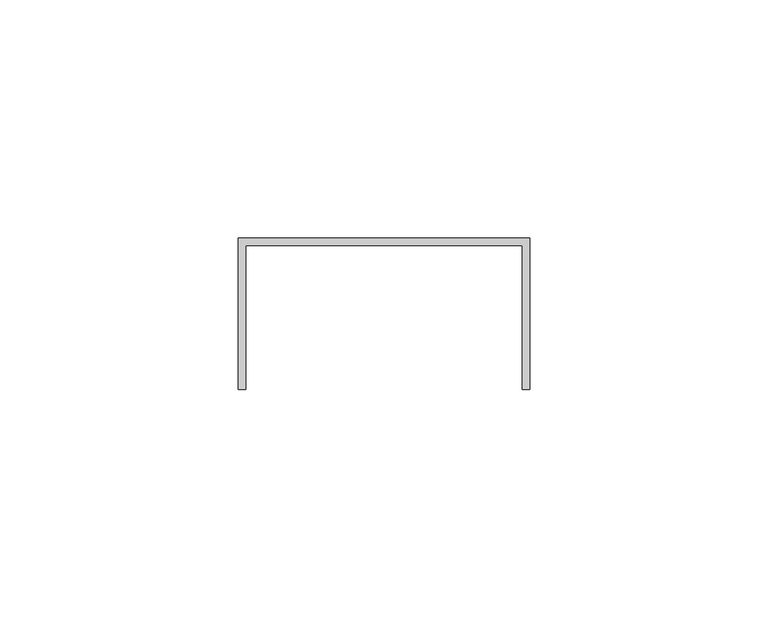
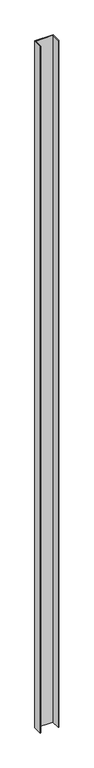
"""IFC4 building model written with IfcOpenShell, lengths in millimetres: proxy geometry, Generic Models 7:Generic Models 1:3:Generic Models 1:3 : Generic Models 7:Generic Models 1:305549:3:Generic Models 1:3:Generic Models 1:3 : Generic Models 7:Generic Models 1:305549:3 : Generic Models 7:Generic Models 1:3:Generic Models 1:3 : Generic Models 7:Generic Models 1:305549:301244:45 : Generic Models 7:Generic Models 1:3:Generic Models 1:3 : Generic Models 7:Generic Models 1:305549:3:Generic Models 1:3:Generic Models 1:3 : Generic Models 7:Generic Models 1:305549:3 : Generic Models 7:Generic Models 1:3:Generic Models 1:3 : Generic Models 7:Generic Models 1:305549:301244:308848."""

import ifcopenshell
import ifcopenshell.guid

model = None  # the IFC model being written
_history = None  # IfcOwnerHistory: only IFC2X3 demands one
_inside = {}  # id of a spatial element -> (the spatial element, [elements in it])
_under = {}  # id of a project, library or spatial element -> (it, [spatial elements below it])
_declared = {}  # id of a project -> (the project, [libraries it declares])
_typed = {}  # id of a type object -> (the type object, [elements of that type])
_made_of = {}  # id of a material, layer set ... -> (it, [elements and type objects made of it])


def new_model(schema):
    """Start an empty IFC model of exactly this schema.

    Asked for "IFC4X3", IfcOpenShell would pick the latest addendum, in which some entities
    have other attributes; the version numbers below select the first issue.
    IFC2X3 requires an IfcOwnerHistory on every rooted entity: one is made here for all.
    """
    global model, _history
    if schema == "IFC4X3":
        model = ifcopenshell.file(schema_version=(4, 3, 0, 0))
    else:
        model = ifcopenshell.file(schema=schema)
    _inside.clear()
    _under.clear()
    _declared.clear()
    _typed.clear()
    _made_of.clear()
    _history = None
    if model.schema == "IFC2X3":
        org = make("IfcOrganization", Name="unknown")
        user = make(
            "IfcPersonAndOrganization",
            ThePerson=make("IfcPerson", FamilyName="unknown"),
            TheOrganization=org,
        )
        app = make(
            "IfcApplication",
            ApplicationDeveloper=org,
            Version="unknown",
            ApplicationFullName="unknown",
            ApplicationIdentifier="unknown",
        )
        _history = make(
            "IfcOwnerHistory",
            OwningUser=user,
            OwningApplication=app,
            ChangeAction="ADDED",
            CreationDate=0,
        )
    return model


def make(cls, **values):
    """One entity of the class cls with the attributes given. An attribute that is None is left unset."""
    return model.create_entity(
        cls, **{name: value for name, value in values.items() if value is not None}
    )


def rooted(cls, **values):
    """An entity with a GlobalId (a new one), such as an element, a storey or a relation."""
    return make(cls, GlobalId=ifcopenshell.guid.new(), OwnerHistory=_history, **values)


def si_unit(unit_type, name, prefix=None):
    """IfcSIUnit, for example si_unit("LENGTHUNIT", "METRE", prefix="MILLI")."""
    return make("IfcSIUnit", UnitType=unit_type, Prefix=prefix, Name=name)


def assignment(units):
    """IfcUnitAssignment: the units of a project."""
    return None if units is None else make("IfcUnitAssignment", Units=units)


def point(xyz):
    """IfcCartesianPoint."""
    return None if xyz is None else make("IfcCartesianPoint", Coordinates=xyz)


def direction(xyz):
    """IfcDirection."""
    return None if xyz is None else make("IfcDirection", DirectionRatios=xyz)


def frame(location, z_axis=None, x_axis=None):
    """IfcAxis2Placement3D, a coordinate frame: its origin and axes. An axis left out is left unset."""
    return make(
        "IfcAxis2Placement3D",
        Location=point(location),
        Axis=direction(z_axis),
        RefDirection=direction(x_axis),
    )


def origin():
    """The frame at (0, 0, 0) with its axes left unset."""
    return frame((0.0, 0.0, 0.0))


def place(relative_to, where):
    """IfcLocalPlacement: puts the frame where relative to a parent placement (None: the world)."""
    return make(
        "IfcLocalPlacement", PlacementRelTo=relative_to, RelativePlacement=where
    )


def context(
    kind, dimensions, precision=None, world=None, true_north=None, identifier=None
):
    """IfcGeometricRepresentationContext, for example the 3D "Model" context."""
    return make(
        "IfcGeometricRepresentationContext",
        ContextIdentifier=identifier,
        ContextType=kind,
        CoordinateSpaceDimension=dimensions,
        Precision=precision,
        WorldCoordinateSystem=world,
        TrueNorth=true_north,
    )


def project(units=None, contexts=None):
    """IfcProject with its units and contexts."""
    return rooted(
        "IfcProject",
        Name="project",
        RepresentationContexts=contexts,
        UnitsInContext=assignment(units),
    )


def spatial(cls, under=None, at=None, **own):
    """A site, building, storey or space (cls), placed at a placement, below another one or the project."""
    s = rooted(cls, ObjectPlacement=at, **own)
    if under is not None:
        _under.setdefault(under.id(), (under, []))[1].append(s)
    return s


def polyline(points):
    """IfcPolyline through the points."""
    return make("IfcPolyline", Points=[point(p) for p in points])


def outline(outer, holes=None, kind="AREA"):
    """IfcArbitraryClosedProfileDef: a profile drawn as a closed curve; with holes, ...WithVoids."""
    if holes is None:
        return make("IfcArbitraryClosedProfileDef", ProfileType=kind, OuterCurve=outer)
    return make(
        "IfcArbitraryProfileDefWithVoids",
        ProfileType=kind,
        OuterCurve=outer,
        InnerCurves=holes,
    )


def extrude(swept, where, along, depth):
    """IfcExtrudedAreaSolid: the profile swept, set in the frame where, extruded along a direction by depth."""
    return make(
        "IfcExtrudedAreaSolid",
        SweptArea=swept,
        Position=where,
        ExtrudedDirection=direction(along),
        Depth=depth,
    )


def shape(context_of_items, identifier, shape_type, items):
    """IfcShapeRepresentation: the items that make up one representation, for example the "Body"."""
    return make(
        "IfcShapeRepresentation",
        ContextOfItems=context_of_items,
        RepresentationIdentifier=identifier,
        RepresentationType=shape_type,
        Items=items,
    )


def source(mapping_origin, context_of_items, identifier, shape_type, items):
    """IfcRepresentationMap: a shape defined once, which mapped items show again and again."""
    return make(
        "IfcRepresentationMap",
        MappingOrigin=mapping_origin,
        MappedRepresentation=shape(context_of_items, identifier, shape_type, items),
    )


def transform(
    local_origin,
    x_axis=None,
    y_axis=None,
    z_axis=None,
    scale=None,
    scale2=None,
    scale3=None,
    uniform=True,
):
    """IfcCartesianTransformationOperator3D, or its non-uniform kind. x_axis, y_axis, z_axis: its Axis1, 2, 3."""
    if uniform:
        return make(
            "IfcCartesianTransformationOperator3D",
            Axis1=direction(x_axis),
            Axis2=direction(y_axis),
            LocalOrigin=point(local_origin),
            Scale=scale,
            Axis3=direction(z_axis),
        )
    return make(
        "IfcCartesianTransformationOperator3DnonUniform",
        Axis1=direction(x_axis),
        Axis2=direction(y_axis),
        LocalOrigin=point(local_origin),
        Scale=scale,
        Axis3=direction(z_axis),
        Scale2=scale2,
        Scale3=scale3,
    )


def mapped(mapping_source, mapping_target):
    """IfcMappedItem: shows the shape of a source again, moved by a transform."""
    return make(
        "IfcMappedItem", MappingSource=mapping_source, MappingTarget=mapping_target
    )


def made_of(thing, what):
    """Note that an element or type object is made of a material, layer set ...; save() writes the relation."""
    if what is not None:
        _made_of.setdefault(what.id(), (what, []))[1].append(thing)
    return thing


def element(
    cls,
    number,
    at=None,
    inside=None,
    cuts=None,
    type_object=None,
    material=None,
    context=None,
    identifier="Body",
    shape_type=None,
    held_by="IfcProductDefinitionShape",
    body=None,
    shapes=None,
    **own,
):
    """One element of the class cls, such as IfcWall. Its Tag is "e" and its number.

    at: its placement. inside: the storey or other place that contains it. cuts: it is an
    opening in that element (IfcRelVoidsElement). A single representation is given by context,
    identifier, shape_type and body (its items); several are given by shapes. held_by: the class
    of the entity that holds the representations. save() writes the other relations.
    """
    e = rooted(cls, Tag="e%d" % number, ObjectPlacement=at, **own)
    if body is not None:
        shapes = [shape(context, identifier, shape_type, body)]
    if shapes is not None:
        e.Representation = make(held_by, Representations=shapes)
    if inside is not None:
        _inside.setdefault(inside.id(), (inside, []))[1].append(e)
    if cuts is not None:
        rooted(
            "IfcRelVoidsElement", RelatingBuildingElement=cuts, RelatedOpeningElement=e
        )
    if type_object is not None:
        _typed.setdefault(type_object.id(), (type_object, []))[1].append(e)
    return made_of(e, material)


def aggregate(whole, parts):
    """IfcRelAggregates: a whole, such as a stair, and the parts it consists of."""
    return rooted("IfcRelAggregates", RelatingObject=whole, RelatedObjects=parts)


def save(model, path):
    """Write the relations noted so far, then the file.

    IfcRelAggregates (storeys below a building ...), IfcRelContainedInSpatialStructure (elements
    in a storey), IfcRelDefinesByType, IfcRelAssociatesMaterial and IfcRelDeclares: one each for
    every whole, place, type object, material and project.
    """
    for whole, parts in _under.values():
        aggregate(whole, parts)
    for where, things in _inside.values():
        rooted(
            "IfcRelContainedInSpatialStructure",
            RelatedElements=things,
            RelatingStructure=where,
        )
    for kind, things in _typed.values():
        rooted("IfcRelDefinesByType", RelatedObjects=things, RelatingType=kind)
    for what, things in _made_of.values():
        rooted("IfcRelAssociatesMaterial", RelatedObjects=things, RelatingMaterial=what)
    for by, libraries in _declared.values():
        rooted("IfcRelDeclares", RelatingContext=by, RelatedDefinitions=libraries)
    model.write(path)


def generic_models_20cf957a(model_context):
    return source(origin(), model_context, "Body", "SweptSolid", [
        extrude(outline(polyline([(667562.3929739, -568253.9540363), (667623.5117239, -568253.9540363), (667623.5117239, -568285.7040363), (667621.9242239, -568285.7040363), (667621.9242239, -568255.5415363), (667563.9804739, -568255.5415363), (667563.9804739, -568285.7040363), (667562.3929739, -568285.7040363), (667562.3929739, -568253.9540363)])), frame((0.0, 0.0, 50.8), z_axis=(0.0, 0.0, 1.0), x_axis=(1.0, 0.0, 0.0)), (0.0, 0.0, 1.0), 2430.9324376),
    ])


if __name__ == "__main__":
    model = new_model("IFC4")
    model_context = context("Model", 3, world=origin())
    ifc_project = project(units=[si_unit("LENGTHUNIT", "METRE", prefix="MILLI")], contexts=[model_context])
    site = spatial("IfcSite", under=ifc_project)
    building = spatial("IfcBuilding", under=site)
    placement = place(None, origin())
    generic_models_shape = generic_models_20cf957a(model_context)
    element("IfcBuildingElementProxy", 1, Name="Generic Models 7:Generic Models 1:3:Generic Models 1:3 : Generic Models 7:Generic Models 1:305549:3:Generic Models 1:3:Generic Models 1:3 : Generic Models 7:Generic Models 1:305549:3 : Generic Models 7:Generic Models 1:3:Generic Models 1:3 : Generic Models 7:Generic Models 1:305549:301244:45 : Generic Models 7:Generic Models 1:3:Generic Models 1:3 : Generic Models 7:Generic Models 1:305549:3:Generic Models 1:3:Generic Models 1:3 : Generic Models 7:Generic Models 1:305549:3 : Generic Models 7:Generic Models 1:3:Generic Models 1:3 : Generic Models 7:Generic Models 1:305549:301244:308848", ObjectType="Generic Models 7:Generic Models 1:3:Generic Models 1:3 : Generic Models 7:Generic Models 1:305549:3:Generic Models 1:3:Generic Models 1:3 : Generic Models 7:Generic Models 1:305549:3 : Generic Models 7:Generic Models 1:3:Generic Models 1:3 : Generic Models 7:Generic Models 1:305549:301244:45 : Generic Models 7:Generic Models 1:3:Generic Models 1:3 : Generic Models 7:Generic Models 1:305549:3:Generic Models 1:3:Generic Models 1:3 : Generic Models 7:Generic Models 1:305549:3 : Generic Models 7:Generic Models 1:3:Generic Models 1:3 : Generic Models 7:Generic Models 1:305549:301244:308848", at=placement, inside=building, context=model_context, shape_type="MappedRepresentation", body=[
        mapped(generic_models_shape, transform((0.0, 0.0, 0.0), x_axis=(1.0, 0.0, 0.0), y_axis=(0.0, 1.0, 0.0), z_axis=(0.0, 0.0, 1.0))),
    ])
    save(model, "model.ifc")

# Revit data of these elements
# Type "Generic Models 7:Generic Models 1:3:Generic Models 1:3 : Generic Models 7:Generic Models 1:305549:3:Generic Models 1:3:Generic Models 1:3 : Generic Models 7:Generic Models 1:305549:3 : Generic Models 7:Generic Models 1:3:Generic Models 1:3 : Generic Models 7:Generic Models 1:305549:301244:45 : Generic Models 7:Generic Models 1:3:Generic Models 1:3 : Generic Models 7:Generic Models 1:305549:3:Generic Models 1:3:Generic Models 1:3 : Generic Models 7:Generic Models 1:305549:3 : Generic Models 7:Generic Models 1:3:Generic Models 1:3 : Generic Models 7:Generic Models 1:305549:301244:308848"
#   NameOverride = "Generic Models 7:Generic Models 1:3:Generic Models 1:3 : Generic Models 7:Generic Models 1:305549:3:Generic Models 1:3:Generic Models 1:3 : Generic Models 7:Generic Models 1:305549:3 : Generic Models 7:Generic Models 1:3:Generic Models 1:3 : Generic Models 7:Generic Models 1:305549:301244:308848"
#   ObjectTypeOverride = "Generic Models 1:3:Generic Models 1:3 : Generic Models 7:Generic Models 1:305549:3 : Generic Models 7:Generic Models 1:3:Generic Models 1:3 : Generic Models 7:Generic Models 1:305549:301244"
#   Reference = "Generic Models 1"
#   Tag = "308848"
# Element 1 (IfcBuildingElementProxy, "Generic Models 7:Generic Models 1:3:Generic Models 1:3 : Generic Models 7:Generic Models 1:305549:3:Generic Models 1:3:Generic Models 1:3 : Generic Models 7:Generic Models 1:305549:3 : Generic Models 7:Generic Models 1:3:Generic Models 1:3 : Generic Models 7:Generic Models 1:305549:301244:45 : Generic Models 7:Generic Models 1:3:Generic Models 1:3 : Generic Models 7:Generic Models 1:305549:3:Generic Models 1:3:Generic Models 1:3 : Generic Models 7:Generic Models 1:305549:3 : Generic Models 7:Generic Models 1:3:Generic Models 1:3 : Generic Models 7:Generic Models 1:305549:301244:308848")
#   Materials on its faces: "GALVANIZED U-CHANNEL (250T125-33)"
# Materials
#   "GALVANIZED U-CHANNEL (250T125-33)": class "Unassigned", colour RGB 202 201 200, transparency 0, Keynote = "M05451300.02", Cost = 0
